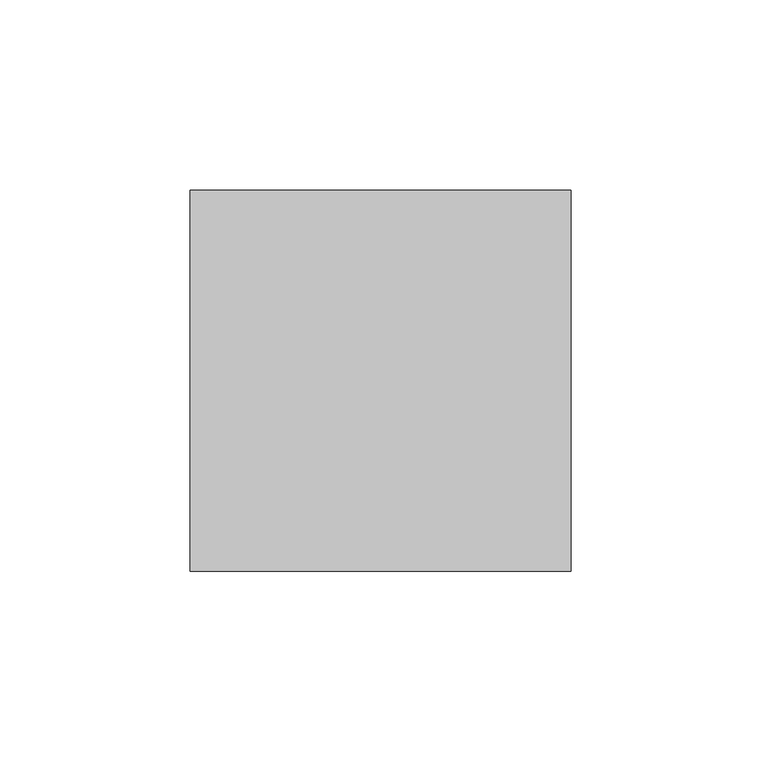
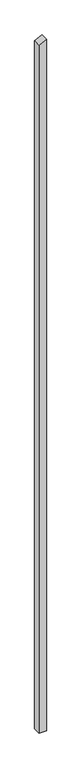
"""IFC4 building model written with IfcOpenShell, lengths in millimetres: column geometry, Holzstütze 158856 : Holzstütze 158856."""

from ifc_helpers import new_model, si_unit, frame, origin, place, context, project, spatial, polyline, outline, extrude, source, transform, mapped, element, save


def column_d1cdecdc(model_context):
    return source(origin(), model_context, "Body", "SweptSolid", [
        extrude(outline(polyline([(-500.0, 163237.7593015), (-500.0, 163337.7593015), (9423.2455407, 163337.7593015), (9372.2929958, 163237.7593015), (-500.0, 163237.7593015)])), frame((0.0, 47884.7962965, 0.0), z_axis=(0.0, 1.0, 0.0), x_axis=(0.0, 0.0, 1.0)), (0.0, 0.0, 1.0), 100.0),
    ])


if __name__ == "__main__":
    model = new_model("IFC4")
    model_context = context("Model", 3, world=origin())
    ifc_project = project(units=[si_unit("LENGTHUNIT", "METRE", prefix="MILLI")], contexts=[model_context])
    site = spatial("IfcSite", under=ifc_project)
    building = spatial("IfcBuilding", under=site)
    placement = place(None, origin())
    column_shape = column_d1cdecdc(model_context)
    element("IfcColumn", 1, ObjectType="Holzstütze 158856 : Holzstütze 158856", at=placement, inside=building, context=model_context, shape_type="MappedRepresentation", body=[
        mapped(column_shape, transform((0.0, 0.0, 0.0), x_axis=(1.0, 0.0, 0.0), y_axis=(0.0, 1.0, 0.0), z_axis=(0.0, 0.0, 1.0))),
    ])
    save(model, "model.ifc")

# Revit data of these elements
# Type "Holzstütze 158856 : Holzstütze 158856"
#   Abrechnungsart = "m"
#   Allright_Bauteil_ID = "0152St 0000143378"
#   Bezeichnung = "Holzstütze"
#   Codetext = "ST-HOLZ\\"
#   Gewerk = "Zimmer- und Holzbauarbeiten"
#   Material = "Holz"
#   Objektname = "Stütze"
#   NameOverride = "Holzstütze"
#   Reference = "Holzstütze"
#   Status = "NEW"
#   ThermalTransmittance = 0.0000 BTU/(h·ft²·°F)
#   Roll = 0.00°
#   Slope = 0.00°
#   2D Interaktion = yes
#   IsExternal = yes
#   LoadBearing = yes
# Element 1 (IfcColumn, "Holzstütze 158856 : Holzstütze 158856")
#   Materials on its faces: "holzschalung"
# Materials
#   "holzschalung": class "Unassigned", colour RGB 128 128 128, transparency 0
